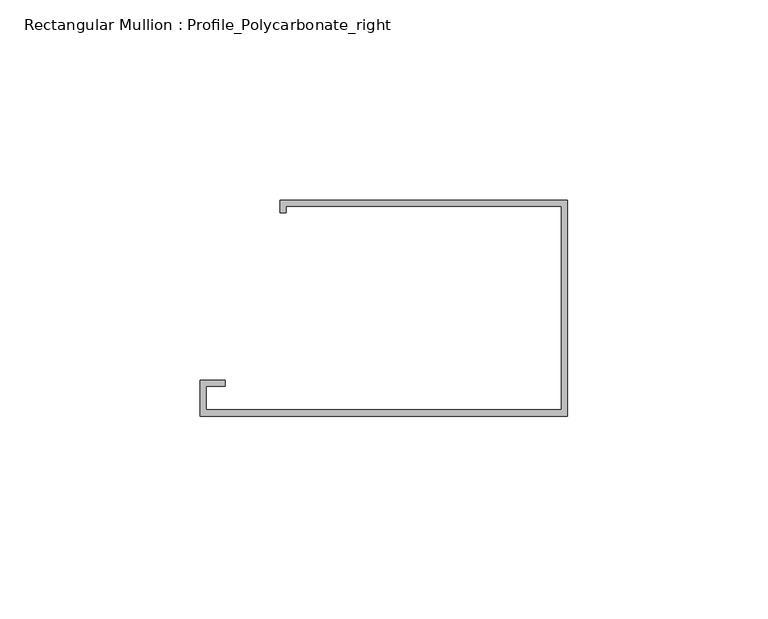
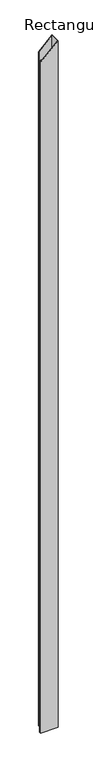
"""IFC4 building model written with IfcOpenShell, lengths in millimetres: member geometry, Rectangular Mullion : Profile_Polycarbonate_right."""

import ifcopenshell
import ifcopenshell.guid

model = None  # the IFC model being written
_history = None  # IfcOwnerHistory: only IFC2X3 demands one
_inside = {}  # id of a spatial element -> (the spatial element, [elements in it])
_under = {}  # id of a project, library or spatial element -> (it, [spatial elements below it])
_declared = {}  # id of a project -> (the project, [libraries it declares])
_typed = {}  # id of a type object -> (the type object, [elements of that type])
_made_of = {}  # id of a material, layer set ... -> (it, [elements and type objects made of it])


def new_model(schema):
    """Start an empty IFC model of exactly this schema.

    Asked for "IFC4X3", IfcOpenShell would pick the latest addendum, in which some entities
    have other attributes; the version numbers below select the first issue.
    IFC2X3 requires an IfcOwnerHistory on every rooted entity: one is made here for all.
    """
    global model, _history
    if schema == "IFC4X3":
        model = ifcopenshell.file(schema_version=(4, 3, 0, 0))
    else:
        model = ifcopenshell.file(schema=schema)
    _inside.clear()
    _under.clear()
    _declared.clear()
    _typed.clear()
    _made_of.clear()
    _history = None
    if model.schema == "IFC2X3":
        org = make("IfcOrganization", Name="unknown")
        user = make(
            "IfcPersonAndOrganization",
            ThePerson=make("IfcPerson", FamilyName="unknown"),
            TheOrganization=org,
        )
        app = make(
            "IfcApplication",
            ApplicationDeveloper=org,
            Version="unknown",
            ApplicationFullName="unknown",
            ApplicationIdentifier="unknown",
        )
        _history = make(
            "IfcOwnerHistory",
            OwningUser=user,
            OwningApplication=app,
            ChangeAction="ADDED",
            CreationDate=0,
        )
    return model


def make(cls, **values):
    """One entity of the class cls with the attributes given. An attribute that is None is left unset."""
    return model.create_entity(
        cls, **{name: value for name, value in values.items() if value is not None}
    )


def rooted(cls, **values):
    """An entity with a GlobalId (a new one), such as an element, a storey or a relation."""
    return make(cls, GlobalId=ifcopenshell.guid.new(), OwnerHistory=_history, **values)


def si_unit(unit_type, name, prefix=None):
    """IfcSIUnit, for example si_unit("LENGTHUNIT", "METRE", prefix="MILLI")."""
    return make("IfcSIUnit", UnitType=unit_type, Prefix=prefix, Name=name)


def assignment(units):
    """IfcUnitAssignment: the units of a project."""
    return None if units is None else make("IfcUnitAssignment", Units=units)


def point(xyz):
    """IfcCartesianPoint."""
    return None if xyz is None else make("IfcCartesianPoint", Coordinates=xyz)


def direction(xyz):
    """IfcDirection."""
    return None if xyz is None else make("IfcDirection", DirectionRatios=xyz)


def frame(location, z_axis=None, x_axis=None):
    """IfcAxis2Placement3D, a coordinate frame: its origin and axes. An axis left out is left unset."""
    return make(
        "IfcAxis2Placement3D",
        Location=point(location),
        Axis=direction(z_axis),
        RefDirection=direction(x_axis),
    )


def origin():
    """The frame at (0, 0, 0) with its axes left unset."""
    return frame((0.0, 0.0, 0.0))


def place(relative_to, where):
    """IfcLocalPlacement: puts the frame where relative to a parent placement (None: the world)."""
    return make(
        "IfcLocalPlacement", PlacementRelTo=relative_to, RelativePlacement=where
    )


def context(
    kind, dimensions, precision=None, world=None, true_north=None, identifier=None
):
    """IfcGeometricRepresentationContext, for example the 3D "Model" context."""
    return make(
        "IfcGeometricRepresentationContext",
        ContextIdentifier=identifier,
        ContextType=kind,
        CoordinateSpaceDimension=dimensions,
        Precision=precision,
        WorldCoordinateSystem=world,
        TrueNorth=true_north,
    )


def project(units=None, contexts=None):
    """IfcProject with its units and contexts."""
    return rooted(
        "IfcProject",
        Name="project",
        RepresentationContexts=contexts,
        UnitsInContext=assignment(units),
    )


def spatial(cls, under=None, at=None, **own):
    """A site, building, storey or space (cls), placed at a placement, below another one or the project."""
    s = rooted(cls, ObjectPlacement=at, **own)
    if under is not None:
        _under.setdefault(under.id(), (under, []))[1].append(s)
    return s


def faces_of(points, faces, orient=None, outer=None):
    """IfcFace entities. A face is a list of loops; a loop is a list of indices into points, from 0.

    orient and outer hold one flag for each loop. By default every Orientation is true, the
    first loop of a face is its IfcFaceOuterBound and the others are IfcFaceBound.
    """
    made = []
    for i, loops in enumerate(faces):
        bounds = []
        for j, loop in enumerate(loops):
            is_outer = j == 0 if outer is None else outer[i][j]
            bounds.append(
                make(
                    "IfcFaceOuterBound" if is_outer else "IfcFaceBound",
                    Bound=make("IfcPolyLoop", Polygon=[points[k] for k in loop]),
                    Orientation=True if orient is None else orient[i][j],
                )
            )
        made.append(make("IfcFace", Bounds=bounds))
    return made


def faceted_brep(points, faces, orient=None, outer=None, voids=None):
    """IfcFacetedBrep: a solid bounded by flat faces; with voids (closed shells), ...WithVoids."""
    shared = [point(p) for p in points]
    hull = make("IfcClosedShell", CfsFaces=faces_of(shared, faces, orient, outer))
    if voids is None:
        return make("IfcFacetedBrep", Outer=hull)
    return make(
        "IfcFacetedBrepWithVoids",
        Outer=hull,
        Voids=[
            make(cls, CfsFaces=faces_of(shared, fs, o, b)) for cls, fs, o, b in voids
        ],
    )


def shape(context_of_items, identifier, shape_type, items):
    """IfcShapeRepresentation: the items that make up one representation, for example the "Body"."""
    return make(
        "IfcShapeRepresentation",
        ContextOfItems=context_of_items,
        RepresentationIdentifier=identifier,
        RepresentationType=shape_type,
        Items=items,
    )


def source(mapping_origin, context_of_items, identifier, shape_type, items):
    """IfcRepresentationMap: a shape defined once, which mapped items show again and again."""
    return make(
        "IfcRepresentationMap",
        MappingOrigin=mapping_origin,
        MappedRepresentation=shape(context_of_items, identifier, shape_type, items),
    )


def transform(
    local_origin,
    x_axis=None,
    y_axis=None,
    z_axis=None,
    scale=None,
    scale2=None,
    scale3=None,
    uniform=True,
):
    """IfcCartesianTransformationOperator3D, or its non-uniform kind. x_axis, y_axis, z_axis: its Axis1, 2, 3."""
    if uniform:
        return make(
            "IfcCartesianTransformationOperator3D",
            Axis1=direction(x_axis),
            Axis2=direction(y_axis),
            LocalOrigin=point(local_origin),
            Scale=scale,
            Axis3=direction(z_axis),
        )
    return make(
        "IfcCartesianTransformationOperator3DnonUniform",
        Axis1=direction(x_axis),
        Axis2=direction(y_axis),
        LocalOrigin=point(local_origin),
        Scale=scale,
        Axis3=direction(z_axis),
        Scale2=scale2,
        Scale3=scale3,
    )


def mapped(mapping_source, mapping_target):
    """IfcMappedItem: shows the shape of a source again, moved by a transform."""
    return make(
        "IfcMappedItem", MappingSource=mapping_source, MappingTarget=mapping_target
    )


def made_of(thing, what):
    """Note that an element or type object is made of a material, layer set ...; save() writes the relation."""
    if what is not None:
        _made_of.setdefault(what.id(), (what, []))[1].append(thing)
    return thing


def element(
    cls,
    number,
    at=None,
    inside=None,
    cuts=None,
    type_object=None,
    material=None,
    context=None,
    identifier="Body",
    shape_type=None,
    held_by="IfcProductDefinitionShape",
    body=None,
    shapes=None,
    **own,
):
    """One element of the class cls, such as IfcWall. Its Tag is "e" and its number.

    at: its placement. inside: the storey or other place that contains it. cuts: it is an
    opening in that element (IfcRelVoidsElement). A single representation is given by context,
    identifier, shape_type and body (its items); several are given by shapes. held_by: the class
    of the entity that holds the representations. save() writes the other relations.
    """
    e = rooted(cls, Tag="e%d" % number, ObjectPlacement=at, **own)
    if body is not None:
        shapes = [shape(context, identifier, shape_type, body)]
    if shapes is not None:
        e.Representation = make(held_by, Representations=shapes)
    if inside is not None:
        _inside.setdefault(inside.id(), (inside, []))[1].append(e)
    if cuts is not None:
        rooted(
            "IfcRelVoidsElement", RelatingBuildingElement=cuts, RelatedOpeningElement=e
        )
    if type_object is not None:
        _typed.setdefault(type_object.id(), (type_object, []))[1].append(e)
    return made_of(e, material)


def aggregate(whole, parts):
    """IfcRelAggregates: a whole, such as a stair, and the parts it consists of."""
    return rooted("IfcRelAggregates", RelatingObject=whole, RelatedObjects=parts)


def save(model, path):
    """Write the relations noted so far, then the file.

    IfcRelAggregates (storeys below a building ...), IfcRelContainedInSpatialStructure (elements
    in a storey), IfcRelDefinesByType, IfcRelAssociatesMaterial and IfcRelDeclares: one each for
    every whole, place, type object, material and project.
    """
    for whole, parts in _under.values():
        aggregate(whole, parts)
    for where, things in _inside.values():
        rooted(
            "IfcRelContainedInSpatialStructure",
            RelatedElements=things,
            RelatingStructure=where,
        )
    for kind, things in _typed.values():
        rooted("IfcRelDefinesByType", RelatedObjects=things, RelatingType=kind)
    for what, things in _made_of.values():
        rooted("IfcRelAssociatesMaterial", RelatedObjects=things, RelatingMaterial=what)
    for by, libraries in _declared.values():
        rooted("IfcRelDeclares", RelatingContext=by, RelatedDefinitions=libraries)
    model.write(path)


def rectangular_mullion_profile_polycarbonate_right_6fadb122(model_context):
    return source(origin(), model_context, "Body", "Brep", [
        faceted_brep([(0.0, -28.984575, -3846.0914015), (-91.9988, -28.984575, -3846.0914015), (-91.9988, -19.992975, -3846.0914015), (-85.6488, -19.992975, -3846.0914015), (-85.6488, -21.580475, -3846.0914015), (-90.4113, -21.580475, -3846.0914015), (-90.4113, -27.397075, -3846.0914015), (-1.5875, -27.397075, -3846.0914015), (-1.5875, 23.428325, -3846.0914015), (-70.3961, 23.428325, -3846.0914015), (-70.3961, 21.840825, -3846.0914015), (-71.9836, 21.840825, -3846.0914015), (-71.9836, 25.015825, -3846.0914015), (0.0, 25.015825, -3846.0914015), (0.0, 25.015825, 0.0), (0.0, -28.984575, 0.0), (-71.9836, 25.015825, -69.046742), (-71.9836, 21.840825, -69.046742), (-70.3961, 21.840825, -67.5240104), (-70.3961, 23.428325, -67.5240104), (-1.5875, 23.428325, -1.5227316), (-1.5875, -27.397075, -1.5227316), (-90.4113, -27.397075, -86.7226105), (-90.4113, -21.580475, -86.7226105), (-85.6488, -21.580475, -82.1544157), (-85.6488, -19.992975, -82.1544157), (-91.9988, -19.992975, -88.2453421), (-91.9988, -28.984575, -88.2453421)], [[[0, 1, 2, 3, 4, 5, 6, 7, 8, 9, 10, 11, 12, 13]], [[14, 15, 0, 13]], [[16, 14, 13, 12]], [[17, 16, 12, 11]], [[18, 17, 11, 10]], [[19, 18, 10, 9]], [[20, 19, 9, 8]], [[21, 20, 8, 7]], [[22, 21, 7, 6]], [[23, 22, 6, 5]], [[24, 23, 5, 4]], [[25, 24, 4, 3]], [[26, 25, 3, 2]], [[27, 26, 2, 1]], [[15, 27, 1, 0]], [[15, 14, 16, 17, 18, 19, 20, 21, 22, 23, 24, 25, 26, 27]]]),
    ])


if __name__ == "__main__":
    model = new_model("IFC4")
    model_context = context("Model", 3, world=origin())
    ifc_project = project(units=[si_unit("LENGTHUNIT", "METRE", prefix="MILLI")], contexts=[model_context])
    site = spatial("IfcSite", under=ifc_project)
    building = spatial("IfcBuilding", under=site)
    placement = place(None, origin())
    rectangular_mullion_profile_polycarbonate_right_shape = rectangular_mullion_profile_polycarbonate_right_6fadb122(model_context)
    element("IfcMember", 1, ObjectType="Rectangular Mullion : Profile_Polycarbonate_right", at=placement, inside=building, context=model_context, shape_type="MappedRepresentation", body=[
        mapped(rectangular_mullion_profile_polycarbonate_right_shape, transform((0.0, 0.0, 0.0), x_axis=(1.0, 0.0, 0.0), y_axis=(0.0, 1.0, 0.0), z_axis=(0.0, 0.0, 1.0))),
    ])
    save(model, "model.ifc")

# Revit data of these elements
# Type "Rectangular Mullion : Profile_Polycarbonate_right"
#   built-in parameter 1007322 = 0.177167 (stored number, unit not read)
#   built-in parameter 1007321 = 0 (stored number, unit not read)
#   built-in parameter 1007320 = 0.00520833 (stored number, unit not read)
